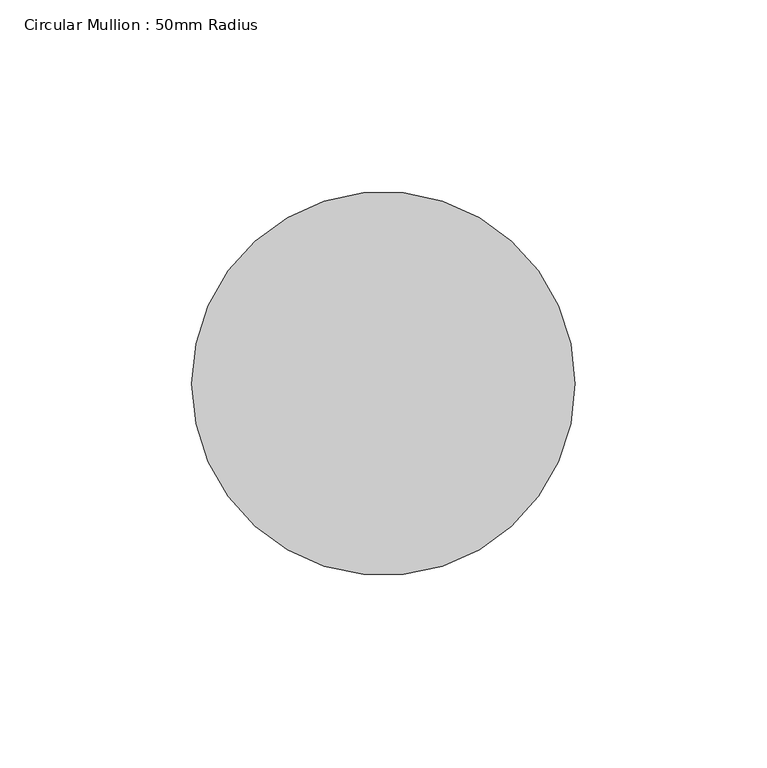
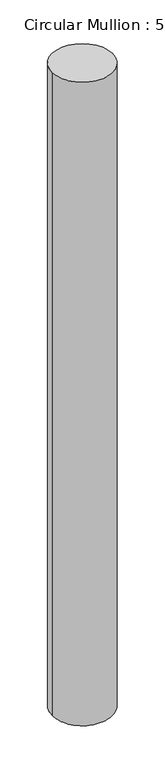
"""IFC4 building model written with IfcOpenShell, lengths in millimetres: member geometry, Circular Mullion : 50mm Radius."""

from ifc_helpers import new_model, si_unit, frame, origin, place, context, project, spatial, ellipse_curve, source, transform, mapped, element, save
from ifc_brep_helpers import plane_surface, cylinder_surface, advanced_brep


def circular_mullion_50mm_radius_291631a5(model_context):
    return source(origin(), model_context, "Body", "AdvancedBrep", [
        advanced_brep(
        [(-100.0, 0.0, 1.6164248), (0.0, 0.0, 0.0), (0.0, 0.0, -1122.1845929), (-100.0, 0.0, -1123.7221469)],
        [
            (0, 1, ellipse_curve(frame((-50.0, 0.0, 0.8082124), z_axis=(-0.01615857198349147, -0.021001264214150158, -0.9996488620775106), x_axis=(-0.6095856226540172, -0.7922772343734078, 0.026498161202963697)), 50.0175631, 50.0)),
            (1, 2),
            (2, 3, ellipse_curve(frame((-50.0, 0.0, -1122.9533699), z_axis=(-0.015370654698110468, -0.01997720966860946, 0.9996822765599118), x_axis=(0.609605998796865, 0.7923037172062775, 0.025206069348310885)), 50.0158912, 50.0)),
            (3, 0),
            (1, 0, ellipse_curve(frame((-50.0, 0.0, 0.8082124), z_axis=(-0.01615857198349147, -0.021001264214150158, -0.9996488620775106), x_axis=(-0.6095856226540172, -0.7922772343734078, 0.026498161202963697)), 50.0175631, 50.0)),
            (3, 2, ellipse_curve(frame((-50.0, 0.0, -1122.9533699), z_axis=(-0.015370654698110468, -0.01997720966860946, 0.9996822765599118), x_axis=(0.609605998796865, 0.7923037172062775, 0.025206069348310885)), 50.0158912, 50.0)),
        ],
        [
            cylinder_surface(frame((-50.0, 0.0, 0.0), z_axis=(0.0, 0.0, 1.0), x_axis=(1.0, 0.0, 0.0)), 50.0),
            plane_surface(frame((-241.5709258, 185.8669627, 0.0), z_axis=(0.01615857198349147, 0.021001264214150158, 0.9996488620775106), x_axis=(0.6095856226540161, 0.7922772343734089, -0.02649816120296311))),
            plane_surface(frame((-241.5709258, 185.8669627, -1122.1845929), z_axis=(0.015370654698110468, 0.01997720966860946, -0.9996822765599118), x_axis=(0.6096059987968648, 0.7923037172062773, 0.025206069348316262))),
        ],
        [
            (0, [[1, 2, 3, 4]]),
            (0, [[5, -4, 6, -2]]),
            (1, [[-1, -5]]),
            (2, [[-6, -3]]),
        ],
    ),
    ])


if __name__ == "__main__":
    model = new_model("IFC4")
    model_context = context("Model", 3, world=origin())
    ifc_project = project(units=[si_unit("LENGTHUNIT", "METRE", prefix="MILLI")], contexts=[model_context])
    site = spatial("IfcSite", under=ifc_project)
    building = spatial("IfcBuilding", under=site)
    placement = place(None, origin())
    circular_mullion_50mm_radius_shape = circular_mullion_50mm_radius_291631a5(model_context)
    element("IfcMember", 1, ObjectType="Circular Mullion : 50mm Radius", at=placement, inside=building, context=model_context, shape_type="MappedRepresentation", body=[
        mapped(circular_mullion_50mm_radius_shape, transform((0.0, 0.0, 0.0), x_axis=(1.0, 0.0, 0.0), y_axis=(0.0, 1.0, 0.0), z_axis=(0.0, 0.0, 1.0))),
    ])
    save(model, "model.ifc")

# Revit data of these elements
# Type "Circular Mullion : 50mm Radius"
#   built-in parameter 1007350 = 0.164042 (stored number, unit not read)
# Element 1 (IfcMember, "Circular Mullion : 50mm Radius")
#   Materials on its faces: "Aluminium"
# Materials
#   "Aluminium": class "Metal", colour RGB 247 247 247, transparency 0, Description = "Aluminium 6061", Cost = 0
